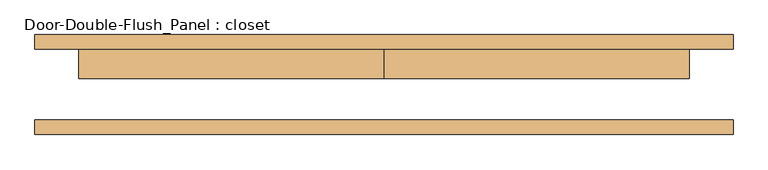
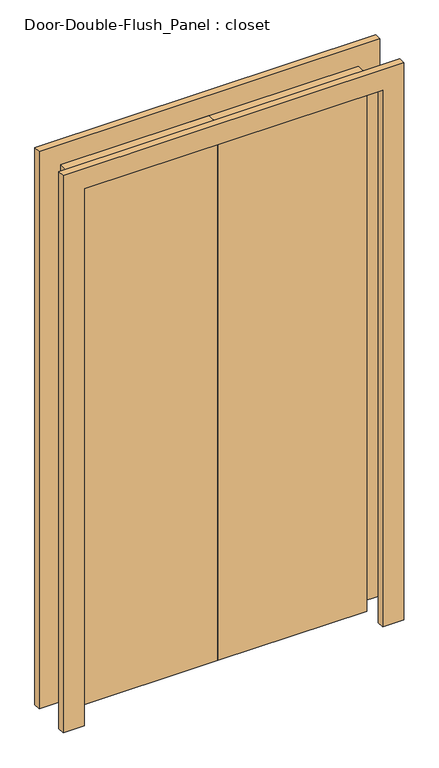
"""IFC4 building model written with IfcOpenShell, lengths in millimetres: door geometry, Door-Double-Flush_Panel : closet."""

from ifc_helpers import new_model, si_unit, frame, origin, origin_with_axes, place, context, project, spatial, polyline, outline, extrude, source, transform, mapped, element, save


def door_double_flush_panel_closet_97aa750d(model_context):
    return source(origin(), model_context, "Body", "SweptSolid", [
        extrude(outline(polyline([(2032.0, -533.4), (2032.0, 533.4), (0.0, 533.4), (0.0, 609.6), (2108.2, 609.6), (2108.2, -609.6), (0.0, -609.6), (0.0, -533.4), (2032.0, -533.4)])), frame((0.0, -87.3125, 0.0), z_axis=(0.0, 1.0, 0.0), x_axis=(0.0, 0.0, 1.0)), (0.0, 0.0, 1.0), 25.4),
        extrude(outline(polyline([(2032.0, -533.4), (2032.0, 533.4), (0.0, 533.4), (0.0, 609.6), (2108.2, 609.6), (2108.2, -609.6), (0.0, -609.6), (0.0, -533.4), (2032.0, -533.4)])), frame((0.0, 61.9125, 0.0), z_axis=(0.0, 1.0, 0.0), x_axis=(0.0, 0.0, 1.0)), (0.0, 0.0, 1.0), 25.4),
        extrude(outline(polyline([(0.0, 61.9125), (533.4, 61.9125), (533.4, 11.1125), (0.0, 11.1125), (0.0, 61.9125)])), origin_with_axes(), (0.0, 0.0, 1.0), 2032.0),
        extrude(outline(polyline([(-533.4, 61.9125), (0.0, 61.9125), (0.0, 11.1125), (-533.4, 11.1125), (-533.4, 61.9125)])), origin_with_axes(), (0.0, 0.0, 1.0), 2032.0),
    ])


if __name__ == "__main__":
    model = new_model("IFC4")
    model_context = context("Model", 3, world=origin())
    ifc_project = project(units=[si_unit("LENGTHUNIT", "METRE", prefix="MILLI")], contexts=[model_context])
    site = spatial("IfcSite", under=ifc_project)
    building = spatial("IfcBuilding", under=site)
    placement = place(None, origin())
    door_double_flush_panel_closet_shape = door_double_flush_panel_closet_97aa750d(model_context)
    element("IfcDoor", 1, ObjectType="Door-Double-Flush_Panel : closet", at=placement, inside=building, context=model_context, shape_type="MappedRepresentation", body=[
        mapped(door_double_flush_panel_closet_shape, transform((0.0, 0.0, 0.0), x_axis=(1.0, 0.0, 0.0), y_axis=(0.0, 1.0, 0.0), z_axis=(0.0, 0.0, 1.0))),
    ])
    save(model, "model.ifc")

# Revit data of these elements
# Type "Door-Double-Flush_Panel : closet"
#   Type Mark = "9"
#   Construction Type Id = "DOOR"
#   Assembly Code = "C1020"
#   Analytic Construction = "Wooden"
#   Thickness = 0' - 2"
#   Thermal Resistance (R) = 0.455703 (m²·K)/W
#   Swing Angle [instance default] = 90.00°
#   Panel Width = 1' - 9"
#   Heat Transfer Coefficient (U) = 2.19465 W/(m²·K)
#   Height = 6' - 8"
#   Trim Projection Ext = 0' - 1"
#   Trim Projection Int = 0' - 1"
#   Trim Width = 0' - 3"
#   Width = 3' - 6"
#   Panel Material = Wood - Birch - Solid Stained Light Low Gloss
#   Trim Material = Paint - Sienna
#   Visual Light Transmittance = 0
#   Solar Heat Gain Coefficient = 0
#   Function = (empty or 0)
#   Wall Closure = (empty or 0)
# Element 1 (IfcDoor, "Door-Double-Flush_Panel : closet")
#   Materials on its faces: "Paint - Sienna", "Wood - Birch - Solid Stained Light Low Gloss"
# Materials
#   "Wood - Birch - Solid Stained Light Low Gloss": class "Wood", colour RGB 210 159 95, transparency 0, Cost = 0
#   "Paint - Sienna": class "Miscellaneous", colour RGB 118 70 51, transparency 0, Cost = 0
